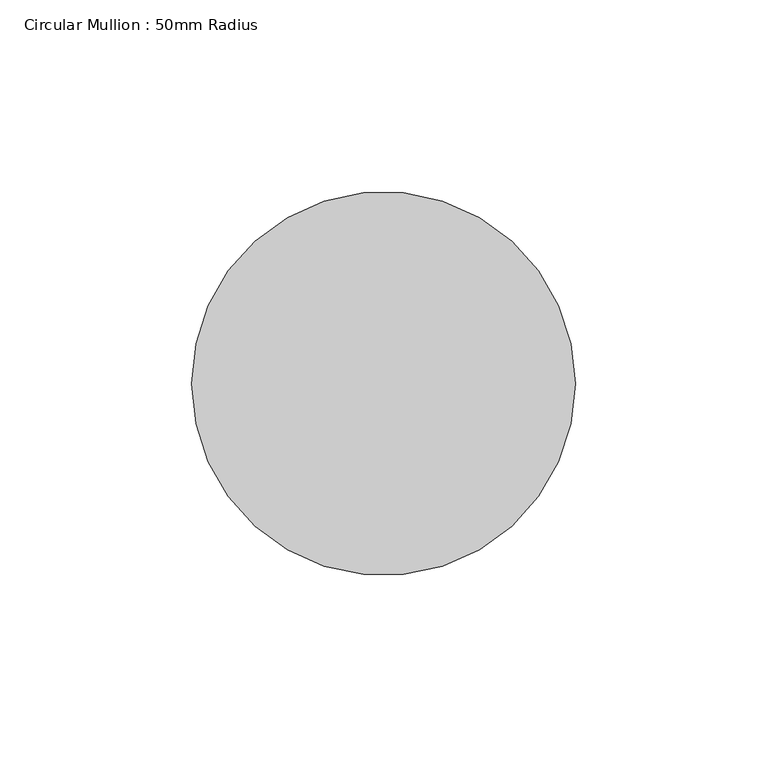
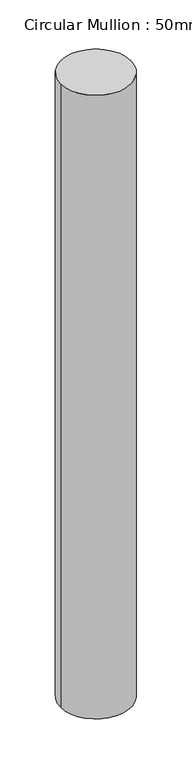
"""IFC4 building model written with IfcOpenShell, lengths in millimetres: member geometry, Circular Mullion : 50mm Radius."""

from ifc_helpers import new_model, si_unit, point, frame, origin, origin_2d, place, context, project, spatial, circle_curve, trimmed, segment, composite_curve, outline, extrude, source, transform, mapped, element, save


def circular_mullion_50mm_radius_b5e21a3a(model_context):
    return source(origin(), model_context, "Body", "SweptSolid", [
        extrude(outline(composite_curve([segment(trimmed(circle_curve(origin_2d(), 50.0), [point((50.0, 0.0))], [point((-50.0, 0.0))], False, "CARTESIAN"), True, "CONTINUOUS"), segment(trimmed(circle_curve(origin_2d(), 50.0), [point((-50.0, 0.0))], [point((50.0, 0.0))], False, "CARTESIAN"), True, "CONTINUOUS")], self_intersect=False)), frame((0.0, 0.0, -939.8373332), z_axis=(0.0, 0.0, 1.0), x_axis=(1.0, 0.0, 0.0)), (0.0, 0.0, 1.0), 939.8373332),
    ])


if __name__ == "__main__":
    model = new_model("IFC4")
    model_context = context("Model", 3, world=origin())
    ifc_project = project(units=[si_unit("LENGTHUNIT", "METRE", prefix="MILLI")], contexts=[model_context])
    site = spatial("IfcSite", under=ifc_project)
    building = spatial("IfcBuilding", under=site)
    placement = place(None, origin())
    circular_mullion_50mm_radius_shape = circular_mullion_50mm_radius_b5e21a3a(model_context)
    element("IfcMember", 1, ObjectType="Circular Mullion : 50mm Radius", at=placement, inside=building, context=model_context, shape_type="MappedRepresentation", body=[
        mapped(circular_mullion_50mm_radius_shape, transform((0.0, 0.0, 0.0), x_axis=(1.0, 0.0, 0.0), y_axis=(0.0, 1.0, 0.0), z_axis=(0.0, 0.0, 1.0))),
    ])
    save(model, "model.ifc")

# Revit data of these elements
# Type "Circular Mullion : 50mm Radius"
#   built-in parameter 1007350 = 0.164042 (stored number, unit not read)
# Element 1 (IfcMember, "Circular Mullion : 50mm Radius")
#   Materials on its faces: "Aluminium"
# Materials
#   "Aluminium": class "Metal", colour RGB 247 247 247, transparency 0, Description = "Aluminium 6061", Cost = 0
